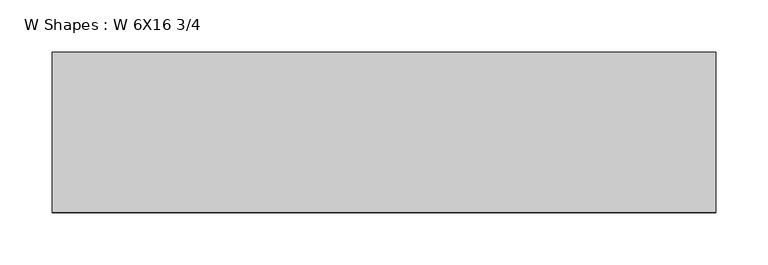
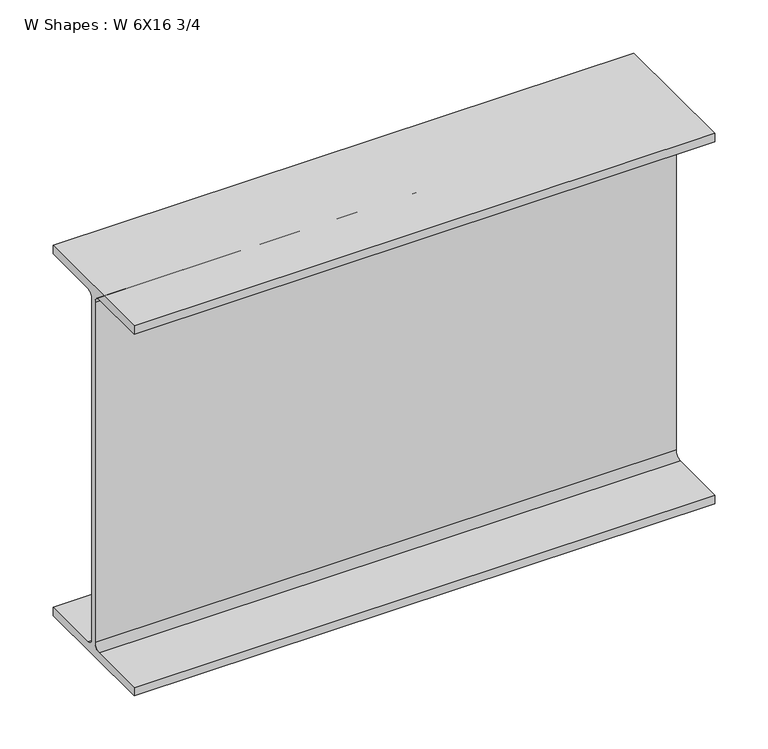
"""IFC4 building model written with IfcOpenShell, lengths in millimetres: beam geometry, W Shapes : W 6X16 3/4."""

from ifc_helpers import new_model, si_unit, point, frame, frame_2d, origin, place, context, project, spatial, polyline, circle_curve, trimmed, segment, composite_curve, outline, extrude, source, transform, mapped, element, save


def w_shapes_w_6x16_3_4_094122b6(model_context):
    return source(origin(), model_context, "Body", "SweptSolid", [
        extrude(outline(composite_curve([segment(polyline([(76.1964281, -203.073), (76.1964281, -212.725), (-76.2035719, -212.725), (-76.2035719, -203.073), (-10.5445719, -203.073)]), True, "CONTINUOUS"), segment(trimmed(circle_curve(frame_2d((-10.5445719, -195.453)), 7.62), [point((-10.5445719, -203.073))], [point((-2.9245719, -195.453))], True, "CARTESIAN"), True, "CONTINUOUS"), segment(polyline([(-2.9245719, -195.453), (-2.9245719, 195.453)]), True, "CONTINUOUS"), segment(trimmed(circle_curve(frame_2d((-10.5445719, 195.453)), 7.62), [point((-2.9245719, 195.453))], [point((-10.5445719, 203.073))], True, "CARTESIAN"), True, "CONTINUOUS"), segment(polyline([(-10.5445719, 203.073), (-76.2035719, 203.073), (-76.2035719, 212.725), (76.1964281, 212.725), (76.1964281, 203.073), (10.5374281, 203.073)]), True, "CONTINUOUS"), segment(trimmed(circle_curve(frame_2d((10.5374281, 195.453)), 7.62), [point((10.5374281, 203.073))], [point((2.9174281, 195.453))], True, "CARTESIAN"), True, "CONTINUOUS"), segment(polyline([(2.9174281, 195.453), (2.9174281, -195.453)]), True, "CONTINUOUS"), segment(trimmed(circle_curve(frame_2d((10.5374281, -195.453)), 7.62), [point((2.9174281, -195.453))], [point((10.5374281, -203.073))], True, "CARTESIAN"), True, "CONTINUOUS"), segment(polyline([(10.5374281, -203.073), (76.1964281, -203.073)]), True, "CONTINUOUS")], self_intersect=False)), frame((-315.8556375, 0.0, 0.0), z_axis=(1.0, 0.0, 0.0), x_axis=(0.0, 1.0, 0.0)), (0.0, 0.0, 1.0), 631.711275),
    ])


if __name__ == "__main__":
    model = new_model("IFC4")
    model_context = context("Model", 3, world=origin())
    ifc_project = project(units=[si_unit("LENGTHUNIT", "METRE", prefix="MILLI")], contexts=[model_context])
    site = spatial("IfcSite", under=ifc_project)
    building = spatial("IfcBuilding", under=site)
    placement = place(None, origin())
    w_shapes_w_6x16_3_4_shape = w_shapes_w_6x16_3_4_094122b6(model_context)
    element("IfcBeam", 1, ObjectType="W Shapes : W 6X16 3/4", at=placement, inside=building, context=model_context, shape_type="MappedRepresentation", body=[
        mapped(w_shapes_w_6x16_3_4_shape, transform((0.0, 0.0, 0.0), x_axis=(1.0, 0.0, 0.0), y_axis=(0.0, 1.0, 0.0), z_axis=(0.0, 0.0, 1.0))),
    ])
    save(model, "model.ifc")

# Revit data of these elements
# Type "W Shapes : W 6X16 3/4"
#   Section Name Key = "W12x26"
#   Assembly Code = "B10"
#   Width = 152.4 mm
#   Web Thickness = 5.842 mm
#   Web Fillet = 7.62 mm
#   Warping Constant = 163001.3 cm⁶
#   Torsional Moment of Inertia = 12.4869 cm⁴
#   Section Area = 7.65 in²
#   Plastic Modulus weak axis = 0.00472801 (stored number, unit not read)
#   Plastic Modulus strong axis = 0.0215278 (stored number, unit not read)
#   Perimeter = 15.0571 m²/m
#   Nominal Weight = 379.441 N/m
#   Moment of Inertia weak axis = 720.08 cm⁴
#   Moment of Inertia strong axis = 8491.12 cm⁴
#   Height = 425.45 mm
#   Flange Thickness = 9.652 mm
#   Elastic Modulus weak axis = 0.00309028 (stored number, unit not read)
#   Elastic Modulus strong axis = 0.0193287 (stored number, unit not read)
#   Centroid Vertical = 212.725 mm
#   Centroid Horizontal = 76.2 mm
#   Length [instance default] = 5' - 0"
#   Structural Material [instance default] = Steel ASTM A992
#   Principal Axes Angle = 0
# Element 1 (IfcBeam, "W Shapes : W 6X16 3/4")
#   Materials on its faces: "Steel ASTM A992"
# Materials
#   "Steel ASTM A992": class "Metal", colour RGB 189 187 185, transparency 0, Description = "Structural steel 50ksi", Cost = 0
